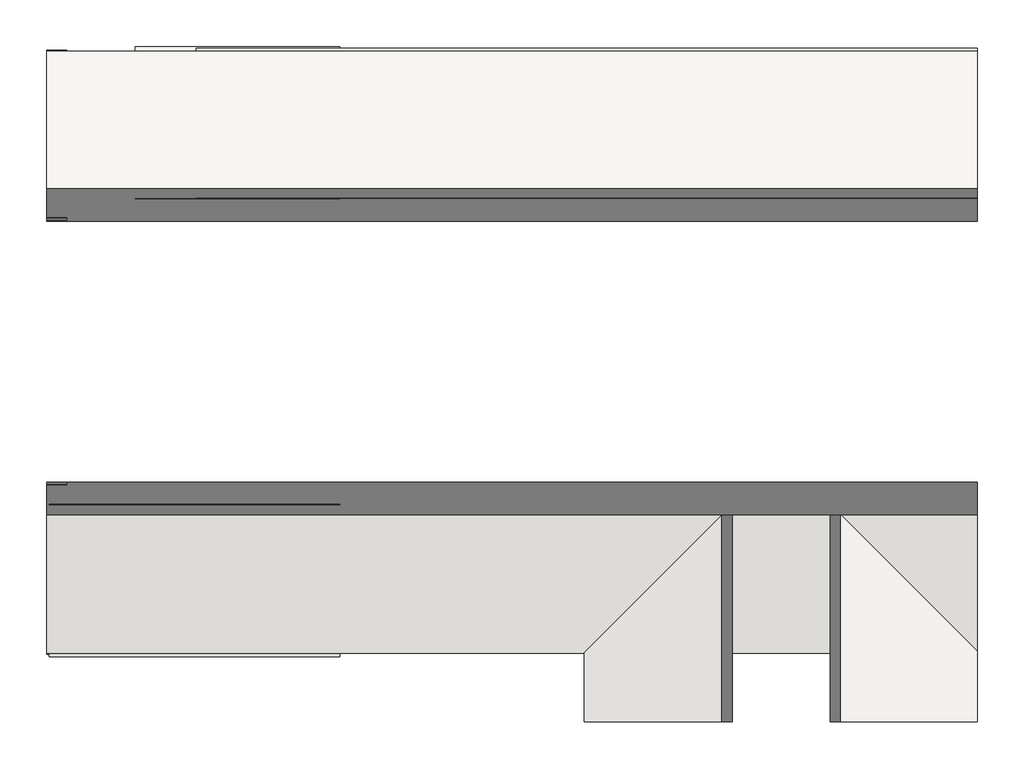
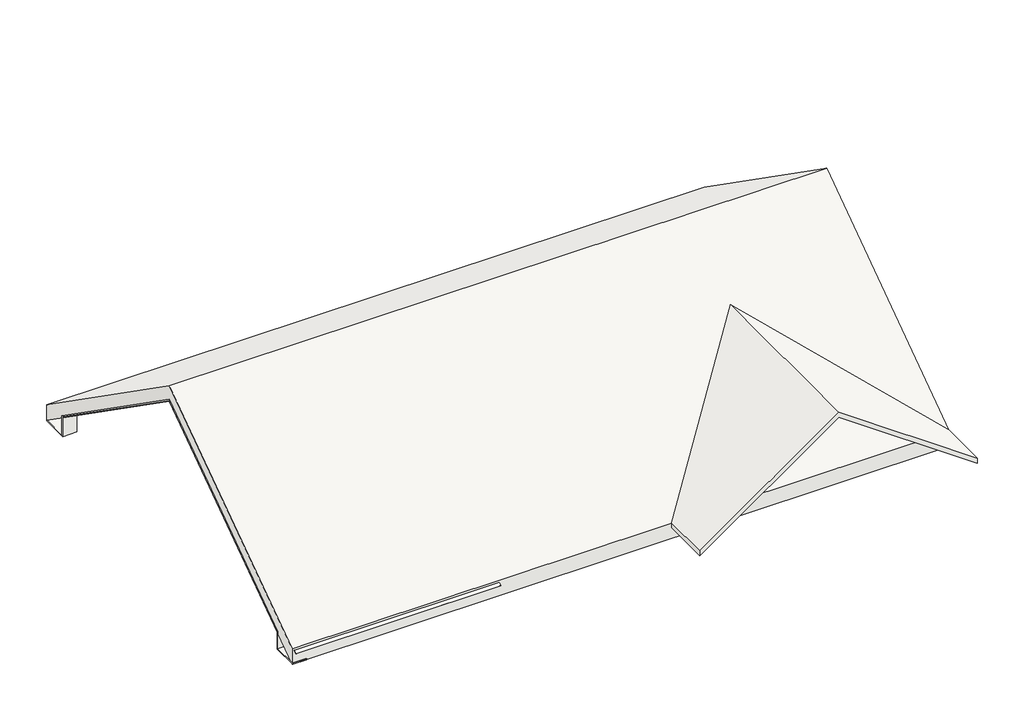
# One storey: 6 roofs.
"""IFC4 building model written with IfcOpenShell, lengths in millimetres."""

import ifcopenshell
import ifcopenshell.guid

model = None  # the IFC model being written
_history = None  # IfcOwnerHistory: only IFC2X3 demands one
_inside = {}  # id of a spatial element -> (the spatial element, [elements in it])
_under = {}  # id of a project, library or spatial element -> (it, [spatial elements below it])
_declared = {}  # id of a project -> (the project, [libraries it declares])
_typed = {}  # id of a type object -> (the type object, [elements of that type])
_made_of = {}  # id of a material, layer set ... -> (it, [elements and type objects made of it])


def new_model(schema):
    """Start an empty IFC model of exactly this schema.

    Asked for "IFC4X3", IfcOpenShell would pick the latest addendum, in which some entities
    have other attributes; the version numbers below select the first issue.
    IFC2X3 requires an IfcOwnerHistory on every rooted entity: one is made here for all.
    """
    global model, _history
    if schema == "IFC4X3":
        model = ifcopenshell.file(schema_version=(4, 3, 0, 0))
    else:
        model = ifcopenshell.file(schema=schema)
    _inside.clear()
    _under.clear()
    _declared.clear()
    _typed.clear()
    _made_of.clear()
    _history = None
    if model.schema == "IFC2X3":
        org = make("IfcOrganization", Name="unknown")
        user = make(
            "IfcPersonAndOrganization",
            ThePerson=make("IfcPerson", FamilyName="unknown"),
            TheOrganization=org,
        )
        app = make(
            "IfcApplication",
            ApplicationDeveloper=org,
            Version="unknown",
            ApplicationFullName="unknown",
            ApplicationIdentifier="unknown",
        )
        _history = make(
            "IfcOwnerHistory",
            OwningUser=user,
            OwningApplication=app,
            ChangeAction="ADDED",
            CreationDate=0,
        )
    return model


def make(cls, **values):
    """One entity of the class cls with the attributes given. An attribute that is None is left unset."""
    return model.create_entity(
        cls, **{name: value for name, value in values.items() if value is not None}
    )


def rooted(cls, **values):
    """An entity with a GlobalId (a new one), such as an element, a storey or a relation."""
    return make(cls, GlobalId=ifcopenshell.guid.new(), OwnerHistory=_history, **values)


def si_unit(unit_type, name, prefix=None):
    """IfcSIUnit, for example si_unit("LENGTHUNIT", "METRE", prefix="MILLI")."""
    return make("IfcSIUnit", UnitType=unit_type, Prefix=prefix, Name=name)


def assignment(units):
    """IfcUnitAssignment: the units of a project."""
    return None if units is None else make("IfcUnitAssignment", Units=units)


def point(xyz):
    """IfcCartesianPoint."""
    return None if xyz is None else make("IfcCartesianPoint", Coordinates=xyz)


def direction(xyz):
    """IfcDirection."""
    return None if xyz is None else make("IfcDirection", DirectionRatios=xyz)


def frame(location, z_axis=None, x_axis=None):
    """IfcAxis2Placement3D, a coordinate frame: its origin and axes. An axis left out is left unset."""
    return make(
        "IfcAxis2Placement3D",
        Location=point(location),
        Axis=direction(z_axis),
        RefDirection=direction(x_axis),
    )


def origin():
    """The frame at (0, 0, 0) with its axes left unset."""
    return frame((0.0, 0.0, 0.0))


def place(relative_to, where):
    """IfcLocalPlacement: puts the frame where relative to a parent placement (None: the world)."""
    return make(
        "IfcLocalPlacement", PlacementRelTo=relative_to, RelativePlacement=where
    )


def context(
    kind, dimensions, precision=None, world=None, true_north=None, identifier=None
):
    """IfcGeometricRepresentationContext, for example the 3D "Model" context."""
    return make(
        "IfcGeometricRepresentationContext",
        ContextIdentifier=identifier,
        ContextType=kind,
        CoordinateSpaceDimension=dimensions,
        Precision=precision,
        WorldCoordinateSystem=world,
        TrueNorth=true_north,
    )


def project(units=None, contexts=None):
    """IfcProject with its units and contexts."""
    return rooted(
        "IfcProject",
        Name="project",
        RepresentationContexts=contexts,
        UnitsInContext=assignment(units),
    )


def spatial(cls, under=None, at=None, **own):
    """A site, building, storey or space (cls), placed at a placement, below another one or the project."""
    s = rooted(cls, ObjectPlacement=at, **own)
    if under is not None:
        _under.setdefault(under.id(), (under, []))[1].append(s)
    return s


def polyline(points):
    """IfcPolyline through the points."""
    return make("IfcPolyline", Points=[point(p) for p in points])


def outline(outer, holes=None, kind="AREA"):
    """IfcArbitraryClosedProfileDef: a profile drawn as a closed curve; with holes, ...WithVoids."""
    if holes is None:
        return make("IfcArbitraryClosedProfileDef", ProfileType=kind, OuterCurve=outer)
    return make(
        "IfcArbitraryProfileDefWithVoids",
        ProfileType=kind,
        OuterCurve=outer,
        InnerCurves=holes,
    )


def extrude(swept, where, along, depth):
    """IfcExtrudedAreaSolid: the profile swept, set in the frame where, extruded along a direction by depth."""
    return make(
        "IfcExtrudedAreaSolid",
        SweptArea=swept,
        Position=where,
        ExtrudedDirection=direction(along),
        Depth=depth,
    )


def faces_of(points, faces, orient=None, outer=None):
    """IfcFace entities. A face is a list of loops; a loop is a list of indices into points, from 0.

    orient and outer hold one flag for each loop. By default every Orientation is true, the
    first loop of a face is its IfcFaceOuterBound and the others are IfcFaceBound.
    """
    made = []
    for i, loops in enumerate(faces):
        bounds = []
        for j, loop in enumerate(loops):
            is_outer = j == 0 if outer is None else outer[i][j]
            bounds.append(
                make(
                    "IfcFaceOuterBound" if is_outer else "IfcFaceBound",
                    Bound=make("IfcPolyLoop", Polygon=[points[k] for k in loop]),
                    Orientation=True if orient is None else orient[i][j],
                )
            )
        made.append(make("IfcFace", Bounds=bounds))
    return made


def faceted_brep(points, faces, orient=None, outer=None, voids=None):
    """IfcFacetedBrep: a solid bounded by flat faces; with voids (closed shells), ...WithVoids."""
    shared = [point(p) for p in points]
    hull = make("IfcClosedShell", CfsFaces=faces_of(shared, faces, orient, outer))
    if voids is None:
        return make("IfcFacetedBrep", Outer=hull)
    return make(
        "IfcFacetedBrepWithVoids",
        Outer=hull,
        Voids=[
            make(cls, CfsFaces=faces_of(shared, fs, o, b)) for cls, fs, o, b in voids
        ],
    )


def shape(context_of_items, identifier, shape_type, items):
    """IfcShapeRepresentation: the items that make up one representation, for example the "Body"."""
    return make(
        "IfcShapeRepresentation",
        ContextOfItems=context_of_items,
        RepresentationIdentifier=identifier,
        RepresentationType=shape_type,
        Items=items,
    )


def made_of(thing, what):
    """Note that an element or type object is made of a material, layer set ...; save() writes the relation."""
    if what is not None:
        _made_of.setdefault(what.id(), (what, []))[1].append(thing)
    return thing


def element(
    cls,
    number,
    at=None,
    inside=None,
    cuts=None,
    type_object=None,
    material=None,
    context=None,
    identifier="Body",
    shape_type=None,
    held_by="IfcProductDefinitionShape",
    body=None,
    shapes=None,
    **own,
):
    """One element of the class cls, such as IfcWall. Its Tag is "e" and its number.

    at: its placement. inside: the storey or other place that contains it. cuts: it is an
    opening in that element (IfcRelVoidsElement). A single representation is given by context,
    identifier, shape_type and body (its items); several are given by shapes. held_by: the class
    of the entity that holds the representations. save() writes the other relations.
    """
    e = rooted(cls, Tag="e%d" % number, ObjectPlacement=at, **own)
    if body is not None:
        shapes = [shape(context, identifier, shape_type, body)]
    if shapes is not None:
        e.Representation = make(held_by, Representations=shapes)
    if inside is not None:
        _inside.setdefault(inside.id(), (inside, []))[1].append(e)
    if cuts is not None:
        rooted(
            "IfcRelVoidsElement", RelatingBuildingElement=cuts, RelatedOpeningElement=e
        )
    if type_object is not None:
        _typed.setdefault(type_object.id(), (type_object, []))[1].append(e)
    return made_of(e, material)


def aggregate(whole, parts):
    """IfcRelAggregates: a whole, such as a stair, and the parts it consists of."""
    return rooted("IfcRelAggregates", RelatingObject=whole, RelatedObjects=parts)


def save(model, path):
    """Write the relations noted so far, then the file.

    IfcRelAggregates (storeys below a building ...), IfcRelContainedInSpatialStructure (elements
    in a storey), IfcRelDefinesByType, IfcRelAssociatesMaterial and IfcRelDeclares: one each for
    every whole, place, type object, material and project.
    """
    for whole, parts in _under.values():
        aggregate(whole, parts)
    for where, things in _inside.values():
        rooted(
            "IfcRelContainedInSpatialStructure",
            RelatedElements=things,
            RelatingStructure=where,
        )
    for kind, things in _typed.values():
        rooted("IfcRelDefinesByType", RelatedObjects=things, RelatingType=kind)
    for what, things in _made_of.values():
        rooted("IfcRelAssociatesMaterial", RelatedObjects=things, RelatingMaterial=what)
    for by, libraries in _declared.values():
        rooted("IfcRelDeclares", RelatingContext=by, RelatedDefinitions=libraries)
    model.write(path)


model = new_model("IFC4")

# Units and contexts
model_context = context("Model", 3, world=origin())
ifc_project = project(units=[si_unit("LENGTHUNIT", "METRE", prefix="MILLI")], contexts=[model_context])

# Site, building, storey
site = spatial("IfcSite", under=ifc_project)
building = spatial("IfcBuilding", under=site)
storey = spatial("IfcBuildingStorey", under=building, Name="04 Top of Wallplate", Elevation=5250.0)

# Roofs
placement = place(None, origin())
element("IfcRoof", 1, ObjectType="Generic_Conc_Tile_Felt_&_Batten_78mm", at=placement, inside=storey, context=model_context, shape_type="Brep", body=[
    faceted_brep([(707.4074327, -1669.6462381, 5202.5013726), (-1849.4872787, -1669.6462381, 6992.8583239), (-4421.5247381, -1669.6462381, 5191.8983063), (-4421.5247381, -1669.6462381, 5096.6778884), (-1849.4872787, -1669.6462381, 6897.637906), (707.4074327, -1669.6462381, 5107.2809546), (707.4074327, -749.0280538, 5202.5013726), (-1849.4872787, 1807.8666576, 6992.8583239), (-4421.5247381, -764.1708018, 5191.8983063), (-4421.5247381, -771.3211386, 5186.8915865), (-4421.5247381, -771.3211386, 5096.6778884), (-4292.6862249, -771.3211386, 5186.8915865), (-1849.4872787, 1671.8778076, 6897.637906), (593.7116674, -771.3211386, 5186.8915865), (707.4074327, -771.3211386, 5107.2809546), (707.4074327, -771.3211386, 5186.8915865)], [[[0, 1, 2, 3, 4, 5]], [[1, 0, 6, 7]], [[2, 1, 7, 8]], [[3, 2, 8, 9, 10]], [[4, 3, 10, 11, 12]], [[5, 4, 12, 13, 14]], [[0, 5, 14, 15, 6]], [[6, 15, 13, 12, 11, 9, 8, 7]], [[15, 14, 13]], [[11, 10, 9]]]),
])
element("IfcRoof", 2, ObjectType="Generic - Barge Soffit", at=placement, inside=storey, context=model_context, shape_type="SweptSolid", body=[
    extrude(outline(polyline([(-785.6829806, 4910.0), (-310.6829806, 4910.0), (-310.6829806, 5237.8153544), (3163.3944218, 7670.3905399), (6591.3330078, 5270.1221014), (6591.3330078, 4894.7047294), (7085.4787302, 4894.7047294), (7085.4787302, 4875.7047294), (6572.3330078, 4875.7047294), (6572.3330078, 5260.2313275), (3163.3944218, 7647.1958227), (-291.6829806, 5227.9245804), (-291.6829806, 4891.0), (-785.6829806, 4891.0), (-785.6829806, 4910.0)])), frame((-11429.0923339, 0.0, 0.0), z_axis=(1.0, 0.0, 0.0), x_axis=(0.0, 1.0, 0.0)), (0.0, 0.0, 1.0), 263.5675957),
])
element("IfcRoof", 3, ObjectType="Generic - EPDM Roof Membrane", at=placement, inside=storey, context=model_context, shape_type="SweptSolid", body=[
    extrude(outline(polyline([(7115.1488778, 5146.8134669), (7115.1488778, 5143.4541616), (7039.7177338, 5181.4613782), (6932.8963896, 5204.534251), (3153.3109274, 7851.0284829), (3089.440846, 7806.3061705), (3089.440846, 7809.9684943), (3153.3109274, 7854.6908067), (6934.121349, 5207.3388489), (7040.7255527, 5184.3128774), (7115.1488778, 5146.8134669)])), frame((-9477.5935928, 0.0, 0.0), z_axis=(1.0, 0.0, 0.0), x_axis=(0.0, 1.0, 0.0)), (0.0, 0.0, 1.0), 10185.0010255),
])
element("IfcRoof", 4, ObjectType="Generic - EPDM Roof Membrane", at=placement, inside=storey, context=model_context, shape_type="SweptSolid", body=[
    extrude(outline(polyline([(-821.3067661, 5109.593127), (-689.5010917, 5198.497177), (-595.8808114, 5220.1111217), (3159.0972164, 7849.3750427), (3215.3756, 7809.9684943), (3215.3756, 7806.3061705), (3159.0972164, 7845.7127189), (-594.6377632, 5217.3191897), (-688.284472, 5195.6991434), (-821.3067661, 5105.9744732), (-821.3067661, 5109.593127)])), frame((-11392.5925673, 0.0, 0.0), z_axis=(1.0, 0.0, 0.0), x_axis=(0.0, 1.0, 0.0)), (0.0, 0.0, 1.0), 3785.0678292),
])
element("IfcRoof", 5, ObjectType="Generic - EPDM Roof Membrane", at=placement, inside=storey, context=model_context, shape_type="SweptSolid", body=[
    extrude(outline(polyline([(7135.6385195, 5109.593127), (7135.6385195, 5105.9744732), (7002.6162254, 5195.6991434), (6908.9695166, 5217.3191897), (3155.234537, 7845.7127189), (3098.9561534, 7806.3061705), (3098.9561534, 7809.9684943), (3155.234537, 7849.3750427), (6910.2125648, 5220.1111217), (7003.8328451, 5198.497177), (7135.6385195, 5109.593127)])), frame((-10269.7454289, 0.0, 0.0), z_axis=(1.0, 0.0, 0.0), x_axis=(0.0, 1.0, 0.0)), (0.0, 0.0, 1.0), 2662.2206908),
])
element("IfcRoof", 6, ObjectType="Roof_38Tile_38Batten_Felt_166Truss", at=placement, inside=storey, context=model_context, shape_type="SweptSolid", body=[
    extrude(outline(polyline([(7076.1554457, 5192.6273509), (7076.1554457, 4894.7583512), (3156.5129138, 7639.3215992), (-771.3211386, 4889.0225869), (-771.3211386, 5186.8915865), (3156.5129138, 7937.1905988), (7076.1554457, 5192.6273509)])), frame((-11429.0923339, 0.0, 0.0), z_axis=(1.0, 0.0, 0.0), x_axis=(0.0, 1.0, 0.0)), (0.0, 0.0, 1.0), 12136.4997666),
])

save(model, "model.ifc")

# Revit data of these elements
# Project information
#   Document_Suitability_Code = "A1"
#   Document_Suitability_Description = "Coordination"
#   Project Issue Date = "26-Jan-21"
#   Project Status = "Project Status"
#   Client Name = "Revit Project"
#   Project Address = "Enter address here"
#   Project Name = "Two Storey House"
#   Project Number = "RARC01"
# Type "Generic_Conc_Tile_Felt_&_Batten_78mm"
#   Layers, outside or top first: 38 mm "Concrete Tile" (function 1); 2 mm "Roofing, EPDM Membrane" (function 2); 38 mm "Softwood, Lumber" (function 2)
# Type "Generic - Barge Soffit"
#   Layers, outside or top first: 19 mm "Timber, Painted, White" (function 1)
# Type "Generic - EPDM Roof Membrane"
#   Layers, outside or top first: 3 mm "Roofing, Tile Membrane" (function 2)
# Type "Roof_38Tile_38Batten_Felt_166Truss"
#   Layers, outside or top first: 38 mm "Concrete Tile" (function 4); 38 mm "Softwood, Lumber" (function 2); 2 mm "Roofing, EPDM Membrane" (function 2); 166 mm "Structure, Wood Truss Joist/Rafter Layer" (function 1)
# Element 1 (IfcRoof, "Generic_Conc_Tile_Felt_&_Batten_78mm")
#   built-in parameter 1001710 = 33615
#   Phase Created = New Construction
#   Materials on its faces: "Softwood, Lumber", "Concrete Tile"
# Element 2 (IfcRoof, "Generic - Barge Soffit")
#   built-in parameter 1001710 = 33615
#   Phase Created = New Construction
#   Materials on its faces: "Timber, Painted, White"
# Elements 3, 4, 5 (IfcRoof, "Generic - EPDM Roof Membrane")
#   built-in parameter 1001710 = 33615
#   Phase Created = New Construction
#   Materials on its faces: "Roofing, Tile Membrane"
# Element 6 (IfcRoof, "Roof_38Tile_38Batten_Felt_166Truss")
#   built-in parameter 1001710 = 33615
#   Phase Created = New Construction
#   Materials on its faces: "Structure, Wood Truss Joist/Rafter Layer", "Concrete Tile"
# Materials
#   "Concrete Tile": class "Wood", colour RGB 90 78 68, transparency 0, Description = "Wood roofing shakes", Cost = 0
#   "Roofing, EPDM Membrane": class "Generic", colour RGB 127 127 127, transparency 0, Description = "EPDM roof membrane", Cost = 0
#   "Softwood, Lumber": class "Wood", colour RGB 205 156 65, transparency 0, Description = "Pinus Echinata", Cost = 0
#   "Timber, Painted, White": class "Wood", colour RGB 255 255 255, transparency 0, Comments = "Rendering appearance not upgraded ", Description = "Timber Barge Board, White Paint Finish", Cost = 0
#   "Roofing, Tile Membrane": class "Generic", colour RGB 75 86 88, transparency 0, Description = "Asphalt saturated felt", Cost = 0
#   "Structure, Wood Truss Joist/Rafter Layer": class "Wood", colour RGB 120 120 120, transparency 0, Description = "Wood trusses, thermal airspace", Cost = 0
